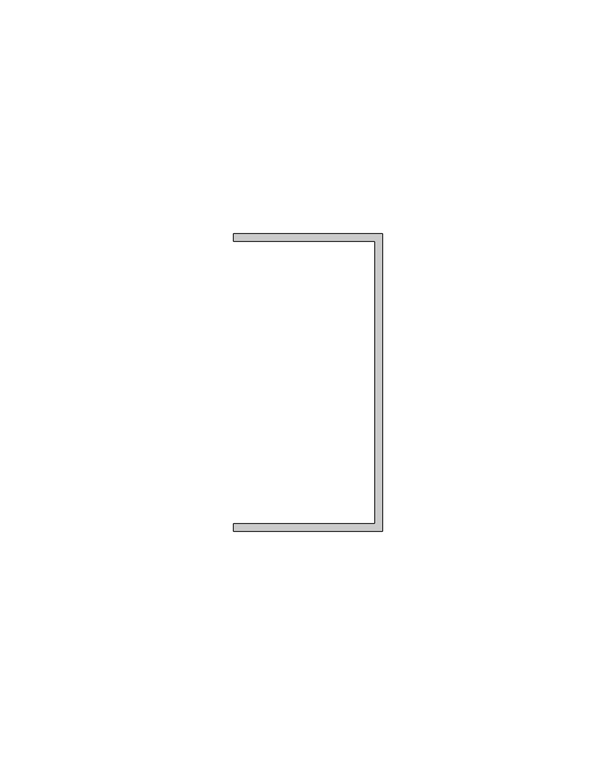
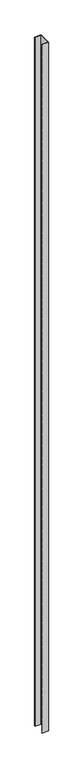
"""IFC4 building model written with IfcOpenShell, lengths in millimetres: proxy geometry, Generic Models 7:Generic Models 1:3:Generic Models 1:3 : Generic Models 7:Generic Models 1:305549:3:Generic Models 1:3:Generic Models 1:3 : Generic Models 7:Generic Models 1:305549:3 : Generic Models 7:Generic Models 1:3:Generic Models 1:3 : Generic Models 7:Generic Models 1:305549:301244:31 : Generic Models 7:Generic Models 1:3:Generic Models 1:3 : Generic Models 7:Generic Models 1:305549:3:Generic Models 1:3:Generic Models 1:3 : Generic Models 7:Generic Models 1:305549:3 : Generic Models 7:Generic Models 1:3:Generic Models 1:3 : Generic Models 7:Generic Models 1:305549:301244:308848."""

from ifc_helpers import new_model, si_unit, frame, origin, place, context, project, spatial, polyline, outline, extrude, source, transform, mapped, element, save


def generic_models_65f7fdad(model_context):
    return source(origin(), model_context, "Body", "SweptSolid", [
        extrude(outline(polyline([(596139.0096495, -579013.3913841), (596139.0096495, -579076.8913841), (596107.2596495, -579076.8913841), (596107.2596495, -579075.3038841), (596137.4221495, -579075.3038841), (596137.4221495, -579014.9788841), (596107.2596495, -579014.9788841), (596107.2596495, -579013.3913841), (596139.0096495, -579013.3913841)])), frame((0.0, 0.0, 38.1), z_axis=(0.0, 0.0, 1.0), x_axis=(1.0, 0.0, 0.0)), (0.0, 0.0, 1.0), 3657.6),
    ])


if __name__ == "__main__":
    model = new_model("IFC4")
    model_context = context("Model", 3, world=origin())
    ifc_project = project(units=[si_unit("LENGTHUNIT", "METRE", prefix="MILLI")], contexts=[model_context])
    site = spatial("IfcSite", under=ifc_project)
    building = spatial("IfcBuilding", under=site)
    placement = place(None, origin())
    generic_models_shape = generic_models_65f7fdad(model_context)
    element("IfcBuildingElementProxy", 1, Name="Generic Models 7:Generic Models 1:3:Generic Models 1:3 : Generic Models 7:Generic Models 1:305549:3:Generic Models 1:3:Generic Models 1:3 : Generic Models 7:Generic Models 1:305549:3 : Generic Models 7:Generic Models 1:3:Generic Models 1:3 : Generic Models 7:Generic Models 1:305549:301244:31 : Generic Models 7:Generic Models 1:3:Generic Models 1:3 : Generic Models 7:Generic Models 1:305549:3:Generic Models 1:3:Generic Models 1:3 : Generic Models 7:Generic Models 1:305549:3 : Generic Models 7:Generic Models 1:3:Generic Models 1:3 : Generic Models 7:Generic Models 1:305549:301244:308848", ObjectType="Generic Models 7:Generic Models 1:3:Generic Models 1:3 : Generic Models 7:Generic Models 1:305549:3:Generic Models 1:3:Generic Models 1:3 : Generic Models 7:Generic Models 1:305549:3 : Generic Models 7:Generic Models 1:3:Generic Models 1:3 : Generic Models 7:Generic Models 1:305549:301244:31 : Generic Models 7:Generic Models 1:3:Generic Models 1:3 : Generic Models 7:Generic Models 1:305549:3:Generic Models 1:3:Generic Models 1:3 : Generic Models 7:Generic Models 1:305549:3 : Generic Models 7:Generic Models 1:3:Generic Models 1:3 : Generic Models 7:Generic Models 1:305549:301244:308848", at=placement, inside=building, context=model_context, shape_type="MappedRepresentation", body=[
        mapped(generic_models_shape, transform((0.0, 0.0, 0.0), x_axis=(1.0, 0.0, 0.0), y_axis=(0.0, 1.0, 0.0), z_axis=(0.0, 0.0, 1.0))),
    ])
    save(model, "model.ifc")

# Revit data of these elements
# Type "Generic Models 7:Generic Models 1:3:Generic Models 1:3 : Generic Models 7:Generic Models 1:305549:3:Generic Models 1:3:Generic Models 1:3 : Generic Models 7:Generic Models 1:305549:3 : Generic Models 7:Generic Models 1:3:Generic Models 1:3 : Generic Models 7:Generic Models 1:305549:301244:31 : Generic Models 7:Generic Models 1:3:Generic Models 1:3 : Generic Models 7:Generic Models 1:305549:3:Generic Models 1:3:Generic Models 1:3 : Generic Models 7:Generic Models 1:305549:3 : Generic Models 7:Generic Models 1:3:Generic Models 1:3 : Generic Models 7:Generic Models 1:305549:301244:308848"
#   NameOverride = "Generic Models 7:Generic Models 1:3:Generic Models 1:3 : Generic Models 7:Generic Models 1:305549:3:Generic Models 1:3:Generic Models 1:3 : Generic Models 7:Generic Models 1:305549:3 : Generic Models 7:Generic Models 1:3:Generic Models 1:3 : Generic Models 7:Generic Models 1:305549:301244:308848"
#   ObjectTypeOverride = "Generic Models 1:3:Generic Models 1:3 : Generic Models 7:Generic Models 1:305549:3 : Generic Models 7:Generic Models 1:3:Generic Models 1:3 : Generic Models 7:Generic Models 1:305549:301244"
#   Reference = "Generic Models 1"
#   Tag = "308848"
# Element 1 (IfcBuildingElementProxy, "Generic Models 7:Generic Models 1:3:Generic Models 1:3 : Generic Models 7:Generic Models 1:305549:3:Generic Models 1:3:Generic Models 1:3 : Generic Models 7:Generic Models 1:305549:3 : Generic Models 7:Generic Models 1:3:Generic Models 1:3 : Generic Models 7:Generic Models 1:305549:301244:31 : Generic Models 7:Generic Models 1:3:Generic Models 1:3 : Generic Models 7:Generic Models 1:305549:3:Generic Models 1:3:Generic Models 1:3 : Generic Models 7:Generic Models 1:305549:3 : Generic Models 7:Generic Models 1:3:Generic Models 1:3 : Generic Models 7:Generic Models 1:305549:301244:308848")
#   Materials on its faces: "GALVANIZED U-CHANNEL (250T125-33)"
# Materials
#   "GALVANIZED U-CHANNEL (250T125-33)": class "Unassigned", colour RGB 202 201 200, transparency 0, Keynote = "M05451300.02", Cost = 0
